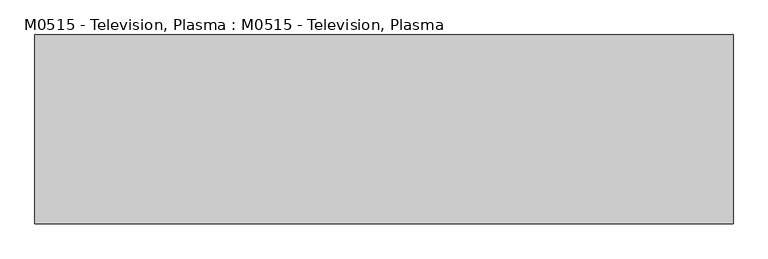
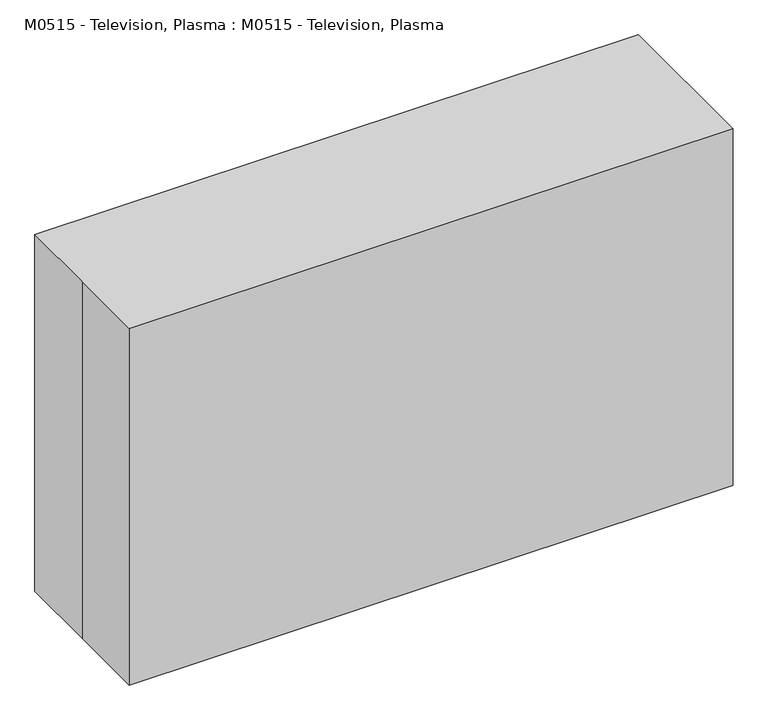
"""IFC4 building model written with IfcOpenShell, lengths in millimetres: proxy geometry, M0515 - Television, Plasma : M0515 - Television, Plasma."""

import ifcopenshell
import ifcopenshell.guid

model = None  # the IFC model being written
_history = None  # IfcOwnerHistory: only IFC2X3 demands one
_inside = {}  # id of a spatial element -> (the spatial element, [elements in it])
_under = {}  # id of a project, library or spatial element -> (it, [spatial elements below it])
_declared = {}  # id of a project -> (the project, [libraries it declares])
_typed = {}  # id of a type object -> (the type object, [elements of that type])
_made_of = {}  # id of a material, layer set ... -> (it, [elements and type objects made of it])


def new_model(schema):
    """Start an empty IFC model of exactly this schema.

    Asked for "IFC4X3", IfcOpenShell would pick the latest addendum, in which some entities
    have other attributes; the version numbers below select the first issue.
    IFC2X3 requires an IfcOwnerHistory on every rooted entity: one is made here for all.
    """
    global model, _history
    if schema == "IFC4X3":
        model = ifcopenshell.file(schema_version=(4, 3, 0, 0))
    else:
        model = ifcopenshell.file(schema=schema)
    _inside.clear()
    _under.clear()
    _declared.clear()
    _typed.clear()
    _made_of.clear()
    _history = None
    if model.schema == "IFC2X3":
        org = make("IfcOrganization", Name="unknown")
        user = make(
            "IfcPersonAndOrganization",
            ThePerson=make("IfcPerson", FamilyName="unknown"),
            TheOrganization=org,
        )
        app = make(
            "IfcApplication",
            ApplicationDeveloper=org,
            Version="unknown",
            ApplicationFullName="unknown",
            ApplicationIdentifier="unknown",
        )
        _history = make(
            "IfcOwnerHistory",
            OwningUser=user,
            OwningApplication=app,
            ChangeAction="ADDED",
            CreationDate=0,
        )
    return model


def make(cls, **values):
    """One entity of the class cls with the attributes given. An attribute that is None is left unset."""
    return model.create_entity(
        cls, **{name: value for name, value in values.items() if value is not None}
    )


def rooted(cls, **values):
    """An entity with a GlobalId (a new one), such as an element, a storey or a relation."""
    return make(cls, GlobalId=ifcopenshell.guid.new(), OwnerHistory=_history, **values)


def si_unit(unit_type, name, prefix=None):
    """IfcSIUnit, for example si_unit("LENGTHUNIT", "METRE", prefix="MILLI")."""
    return make("IfcSIUnit", UnitType=unit_type, Prefix=prefix, Name=name)


def assignment(units):
    """IfcUnitAssignment: the units of a project."""
    return None if units is None else make("IfcUnitAssignment", Units=units)


def point(xyz):
    """IfcCartesianPoint."""
    return None if xyz is None else make("IfcCartesianPoint", Coordinates=xyz)


def direction(xyz):
    """IfcDirection."""
    return None if xyz is None else make("IfcDirection", DirectionRatios=xyz)


def frame(location, z_axis=None, x_axis=None):
    """IfcAxis2Placement3D, a coordinate frame: its origin and axes. An axis left out is left unset."""
    return make(
        "IfcAxis2Placement3D",
        Location=point(location),
        Axis=direction(z_axis),
        RefDirection=direction(x_axis),
    )


def origin():
    """The frame at (0, 0, 0) with its axes left unset."""
    return frame((0.0, 0.0, 0.0))


def origin_with_axes():
    """The frame at (0, 0, 0) with the z axis (0, 0, 1) and the x axis (1, 0, 0) written out."""
    return frame((0.0, 0.0, 0.0), z_axis=(0.0, 0.0, 1.0), x_axis=(1.0, 0.0, 0.0))


def place(relative_to, where):
    """IfcLocalPlacement: puts the frame where relative to a parent placement (None: the world)."""
    return make(
        "IfcLocalPlacement", PlacementRelTo=relative_to, RelativePlacement=where
    )


def context(
    kind, dimensions, precision=None, world=None, true_north=None, identifier=None
):
    """IfcGeometricRepresentationContext, for example the 3D "Model" context."""
    return make(
        "IfcGeometricRepresentationContext",
        ContextIdentifier=identifier,
        ContextType=kind,
        CoordinateSpaceDimension=dimensions,
        Precision=precision,
        WorldCoordinateSystem=world,
        TrueNorth=true_north,
    )


def project(units=None, contexts=None):
    """IfcProject with its units and contexts."""
    return rooted(
        "IfcProject",
        Name="project",
        RepresentationContexts=contexts,
        UnitsInContext=assignment(units),
    )


def spatial(cls, under=None, at=None, **own):
    """A site, building, storey or space (cls), placed at a placement, below another one or the project."""
    s = rooted(cls, ObjectPlacement=at, **own)
    if under is not None:
        _under.setdefault(under.id(), (under, []))[1].append(s)
    return s


def polyline(points):
    """IfcPolyline through the points."""
    return make("IfcPolyline", Points=[point(p) for p in points])


def outline(outer, holes=None, kind="AREA"):
    """IfcArbitraryClosedProfileDef: a profile drawn as a closed curve; with holes, ...WithVoids."""
    if holes is None:
        return make("IfcArbitraryClosedProfileDef", ProfileType=kind, OuterCurve=outer)
    return make(
        "IfcArbitraryProfileDefWithVoids",
        ProfileType=kind,
        OuterCurve=outer,
        InnerCurves=holes,
    )


def extrude(swept, where, along, depth):
    """IfcExtrudedAreaSolid: the profile swept, set in the frame where, extruded along a direction by depth."""
    return make(
        "IfcExtrudedAreaSolid",
        SweptArea=swept,
        Position=where,
        ExtrudedDirection=direction(along),
        Depth=depth,
    )


def shape(context_of_items, identifier, shape_type, items):
    """IfcShapeRepresentation: the items that make up one representation, for example the "Body"."""
    return make(
        "IfcShapeRepresentation",
        ContextOfItems=context_of_items,
        RepresentationIdentifier=identifier,
        RepresentationType=shape_type,
        Items=items,
    )


def source(mapping_origin, context_of_items, identifier, shape_type, items):
    """IfcRepresentationMap: a shape defined once, which mapped items show again and again."""
    return make(
        "IfcRepresentationMap",
        MappingOrigin=mapping_origin,
        MappedRepresentation=shape(context_of_items, identifier, shape_type, items),
    )


def transform(
    local_origin,
    x_axis=None,
    y_axis=None,
    z_axis=None,
    scale=None,
    scale2=None,
    scale3=None,
    uniform=True,
):
    """IfcCartesianTransformationOperator3D, or its non-uniform kind. x_axis, y_axis, z_axis: its Axis1, 2, 3."""
    if uniform:
        return make(
            "IfcCartesianTransformationOperator3D",
            Axis1=direction(x_axis),
            Axis2=direction(y_axis),
            LocalOrigin=point(local_origin),
            Scale=scale,
            Axis3=direction(z_axis),
        )
    return make(
        "IfcCartesianTransformationOperator3DnonUniform",
        Axis1=direction(x_axis),
        Axis2=direction(y_axis),
        LocalOrigin=point(local_origin),
        Scale=scale,
        Axis3=direction(z_axis),
        Scale2=scale2,
        Scale3=scale3,
    )


def mapped(mapping_source, mapping_target):
    """IfcMappedItem: shows the shape of a source again, moved by a transform."""
    return make(
        "IfcMappedItem", MappingSource=mapping_source, MappingTarget=mapping_target
    )


def made_of(thing, what):
    """Note that an element or type object is made of a material, layer set ...; save() writes the relation."""
    if what is not None:
        _made_of.setdefault(what.id(), (what, []))[1].append(thing)
    return thing


def element(
    cls,
    number,
    at=None,
    inside=None,
    cuts=None,
    type_object=None,
    material=None,
    context=None,
    identifier="Body",
    shape_type=None,
    held_by="IfcProductDefinitionShape",
    body=None,
    shapes=None,
    **own,
):
    """One element of the class cls, such as IfcWall. Its Tag is "e" and its number.

    at: its placement. inside: the storey or other place that contains it. cuts: it is an
    opening in that element (IfcRelVoidsElement). A single representation is given by context,
    identifier, shape_type and body (its items); several are given by shapes. held_by: the class
    of the entity that holds the representations. save() writes the other relations.
    """
    e = rooted(cls, Tag="e%d" % number, ObjectPlacement=at, **own)
    if body is not None:
        shapes = [shape(context, identifier, shape_type, body)]
    if shapes is not None:
        e.Representation = make(held_by, Representations=shapes)
    if inside is not None:
        _inside.setdefault(inside.id(), (inside, []))[1].append(e)
    if cuts is not None:
        rooted(
            "IfcRelVoidsElement", RelatingBuildingElement=cuts, RelatedOpeningElement=e
        )
    if type_object is not None:
        _typed.setdefault(type_object.id(), (type_object, []))[1].append(e)
    return made_of(e, material)


def aggregate(whole, parts):
    """IfcRelAggregates: a whole, such as a stair, and the parts it consists of."""
    return rooted("IfcRelAggregates", RelatingObject=whole, RelatedObjects=parts)


def save(model, path):
    """Write the relations noted so far, then the file.

    IfcRelAggregates (storeys below a building ...), IfcRelContainedInSpatialStructure (elements
    in a storey), IfcRelDefinesByType, IfcRelAssociatesMaterial and IfcRelDeclares: one each for
    every whole, place, type object, material and project.
    """
    for whole, parts in _under.values():
        aggregate(whole, parts)
    for where, things in _inside.values():
        rooted(
            "IfcRelContainedInSpatialStructure",
            RelatedElements=things,
            RelatingStructure=where,
        )
    for kind, things in _typed.values():
        rooted("IfcRelDefinesByType", RelatedObjects=things, RelatingType=kind)
    for what, things in _made_of.values():
        rooted("IfcRelAssociatesMaterial", RelatedObjects=things, RelatingMaterial=what)
    for by, libraries in _declared.values():
        rooted("IfcRelDeclares", RelatingContext=by, RelatedDefinitions=libraries)
    model.write(path)


def m0515_television_plasma_m0515_television_plasma_2e7fd35f(model_context):
    return source(origin(), model_context, "Body", "SweptSolid", [
        extrude(outline(polyline([(-490.2983915, -38.1), (-541.0983915, -38.1), (-541.0983915, 0.0), (-490.2983915, 0.0), (-490.2983915, -38.1)])), frame((0.0, 0.0, 101.6), z_axis=(0.0, 0.0, 1.0), x_axis=(1.0, 0.0, 0.0)), (0.0, 0.0, 1.0), 573.8106904),
        extrude(outline(polyline([(541.0983915, -38.1), (490.2983915, -38.1), (490.2983915, 0.0), (541.0983915, 0.0), (541.0983915, -38.1)])), frame((0.0, 0.0, 101.6), z_axis=(0.0, 0.0, 1.0), x_axis=(1.0, 0.0, 0.0)), (0.0, 0.0, 1.0), 573.8106904),
        extrude(outline(polyline([(675.4106904, 490.2983915), (675.4106904, -490.2983915), (101.6, -490.2983915), (101.6, 490.2983915), (675.4106904, 490.2983915)]), holes=[polyline([(650.0106904, 464.8983915), (127.0, 464.8983915), (127.0, -464.8983915), (650.0106904, -464.8983915), (650.0106904, 464.8983915)])]), frame((0.0, -38.1, 0.0), z_axis=(0.0, 1.0, 0.0), x_axis=(0.0, 0.0, 1.0)), (0.0, 0.0, 1.0), 76.2),
        extrude(outline(polyline([(464.8983915, -12.7), (-464.8983915, -12.7), (-464.8983915, 38.1), (464.8983915, 38.1), (464.8983915, -12.7)])), frame((0.0, 0.0, 127.0), z_axis=(0.0, 0.0, 1.0), x_axis=(1.0, 0.0, 0.0)), (0.0, 0.0, 1.0), 523.0106904),
        extrude(outline(polyline([(-609.6, 165.1), (609.6, 165.1), (609.6, -165.1), (-609.6, -165.1), (-609.6, 0.0), (-609.6, 165.1)])), origin_with_axes(), (0.0, 0.0, 1.0), 762.0),
    ])


if __name__ == "__main__":
    model = new_model("IFC4")
    model_context = context("Model", 3, world=origin())
    ifc_project = project(units=[si_unit("LENGTHUNIT", "METRE", prefix="MILLI")], contexts=[model_context])
    site = spatial("IfcSite", under=ifc_project)
    building = spatial("IfcBuilding", under=site)
    placement = place(None, origin())
    m0515_television_plasma_m0515_television_plasma_shape = m0515_television_plasma_m0515_television_plasma_2e7fd35f(model_context)
    element("IfcBuildingElementProxy", 1, Name="M0515 - Television, Plasma : M0515 - Television, Plasma", ObjectType="M0515 - Television, Plasma : M0515 - Television, Plasma", at=placement, inside=building, context=model_context, shape_type="MappedRepresentation", body=[
        mapped(m0515_television_plasma_m0515_television_plasma_shape, transform((0.0, 0.0, 0.0), x_axis=(1.0, 0.0, 0.0), y_axis=(0.0, 1.0, 0.0), z_axis=(0.0, 0.0, 1.0))),
    ])
    save(model, "model.ifc")

# Revit data of these elements
# Type "M0515 - Television, Plasma : M0515 - Television, Plasma"
#   Watts2 = "0"
#   Watts1 = "360"
#   Unit_Issue = "EA"
#   UTIL_6_Misc = "A"
#   UTIL_5_NonMedGas = "-"
#   UTIL_4_MiscGas = "-"
#   UTIL_3_MedGas = "-"
#   UTIL_2_Elec = "A"
#   UTIL_1_WaterDrain = "-"
#   Nomenclature = "Television, Plasma"
#   NSN = ""
#   Location [instance default] = ""
#   JSN = "M0515"
#   Fund_Source_VA = "-"
#   Fund_Source_Navy = "-"
#   Fund_Source_Army = "-"
#   Fund_Source_AF = "-"
#   ELEC_Volts2 = "0"
#   ELEC_Volts1 = "120"
#   ELEC_Phase2 = "0"
#   ELEC_Phase1 = "1"
#   ELEC_HertzSwitch = "0"
#   ELEC_HertzDependent = "-1"
#   ELEC_Hertz = "60"
#   ELEC_Amps2 = "0"
#   ELEC_Amps1 = "3"
#   DetailDescription = "42\" diagonal screen, high definition (HDTV) multimedia flat panel plasma display television. The TV will have a 16:9 wide screen aspect ratio, a minimum of 1024 x 768 display resolution, NTSC tuner, built-in stereo speakers and surround sound."
#   CAT_VA = "C"
#   CAT_Navy = "C"
#   CAT_IHS = "-"
#   CAT_Army = "C"
#   CAT_AF = "C"
#   BTUperhour = "0"
#   Weight_IP = 95
#   DIM_Width_IP = 4' - 0"
#   DIM_Height_IP = 2' - 6"
#   DIM_Depth_IP = 1' - 1"
# Element 1 (IfcBuildingElementProxy, "M0515 - Television, Plasma : M0515 - Television, Plasma")
#   Materials on its faces: "EquipSpace"
# Materials
#   "EquipSpace": class "Unassigned", colour RGB 221 217 195, transparency 0.5
